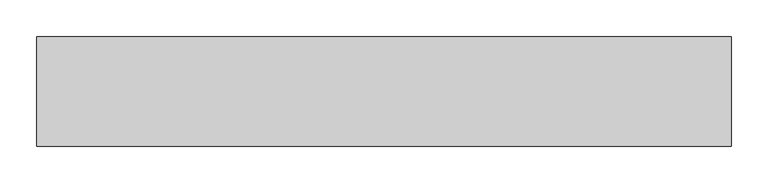
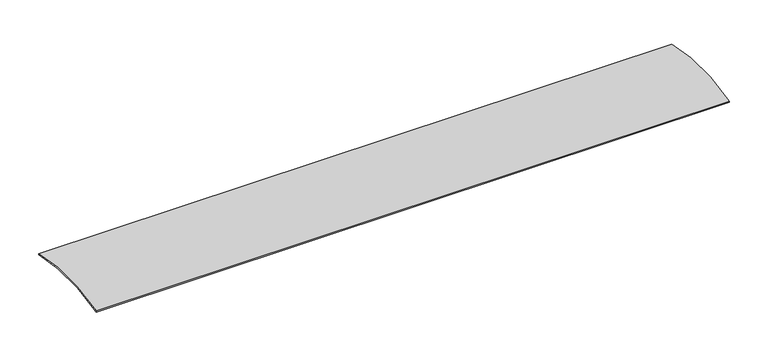
"""IFC4 building model written with IfcOpenShell, lengths in millimetres: proxy geometry, TN_ПВС 125-82_Защитная решетка : TN_ПВС 125-82_Защитная решетка."""

from ifc_helpers import new_model, si_unit, point, frame, frame_2d, origin, place, context, project, spatial, polyline, circle_curve, trimmed, segment, composite_curve, outline, extrude, source, transform, mapped, element, save


def generic_models_7c3ca5dc(model_context):
    return source(origin(), model_context, "Body", "SweptSolid", [
        extrude(outline(composite_curve([segment(polyline([(-74.1, -0.0644007), (-74.1, 2.0)]), True, "CONTINUOUS"), segment(trimmed(circle_curve(frame_2d((0.0, -288.7046439)), 300.0), [point((-74.1, 2.0))], [point((74.1, 2.0))], False, "CARTESIAN"), True, "CONTINUOUS"), segment(polyline([(74.1, 2.0), (74.1, -0.0644007)]), True, "CONTINUOUS"), segment(trimmed(circle_curve(frame_2d((0.0, -288.7046439)), 298.0), [point((74.1, -0.0644007))], [point((-74.1, -0.0644007))], True, "CARTESIAN"), True, "CONTINUOUS")], self_intersect=False)), frame((0.0, 0.0, 0.0), z_axis=(1.0, 0.0, 0.0), x_axis=(0.0, 1.0, 0.0)), (0.0, 0.0, 1.0), 942.0),
    ])


if __name__ == "__main__":
    model = new_model("IFC4")
    model_context = context("Model", 3, world=origin())
    ifc_project = project(units=[si_unit("LENGTHUNIT", "METRE", prefix="MILLI")], contexts=[model_context])
    site = spatial("IfcSite", under=ifc_project)
    building = spatial("IfcBuilding", under=site)
    placement = place(None, origin())
    generic_models_shape = generic_models_7c3ca5dc(model_context)
    element("IfcBuildingElementProxy", 1, Name="TN_ПВС 125-82_Защитная решетка : TN_ПВС 125-82_Защитная решетка", ObjectType="TN_ПВС 125-82_Защитная решетка : TN_ПВС 125-82_Защитная решетка", at=placement, inside=building, context=model_context, shape_type="MappedRepresentation", body=[
        mapped(generic_models_shape, transform((0.0, 0.0, 0.0), x_axis=(1.0, 0.0, 0.0), y_axis=(0.0, 1.0, 0.0), z_axis=(0.0, 0.0, 1.0))),
    ])
    save(model, "model.ifc")

# Revit data of these elements
# Type "TN_ПВС 125-82_Защитная решетка : TN_ПВС 125-82_Защитная решетка"
#   Description = "Служит для предотвращения засора водосточной системы. Не пропускает в желоб листья и прочий крупный\r\nмусор"
#   Manufacturer = "ТехноНИКОЛЬ"
#   Model = "Комплектующие к водосточным системам"
#   URL = "https://tn-vodostok.ru/catalog/pvh/"
#   ADSK_Обозначение = "ТехноНИКОЛЬ"
#   ADSK_Наименование краткое = "Решетка"
#   ADSK_Наименование = "Защитная решетка"
#   ADSK_Масса_Текст = ""
#   ADSK_Марка = ""
#   ADSK_Код изделия = ""
#   ADSK_Завод-изготовитель = "ТехноНИКОЛЬ"
#   ADSK_Единица измерения = "п.м."
#   ADSK_Группирование = "Комплектующие к водосточным системам"
#   ADSK_URL страницы изделия = "https://tn-vodostok.ru/catalog/pvh/"
#   ADSK_URL документации изделия = "https://tn-vodostok.ru/upload/iblock/c42/c427963cb77eb5c3c51f0cfb870e9e52.pdf"
#   ADSK_Размер_Длина [instance default] = 500 mm
#   ADSK_Количество [instance default] = 0.5
#   ADSK_Материал [instance default] = TN_Пластик_Решетка_Коричневый_RAL8019
#   Default Elevation = 0
# Element 1 (IfcBuildingElementProxy, "TN_ПВС 125-82_Защитная решетка : TN_ПВС 125-82_Защитная решетка")
#   ADSK_Размер_Длина = 942 mm
#   ADSK_Количество = 0.942
#   Materials on its faces: "TN_Пластик_Решетка_Коричневый_RAL8019"
# Materials
#   "TN_Пластик_Решетка_Коричневый_RAL8019": class "Типовые", colour RGB 61 54 53, transparency 0.25, Cost = 0
